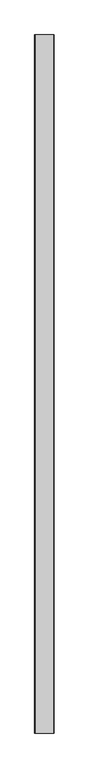
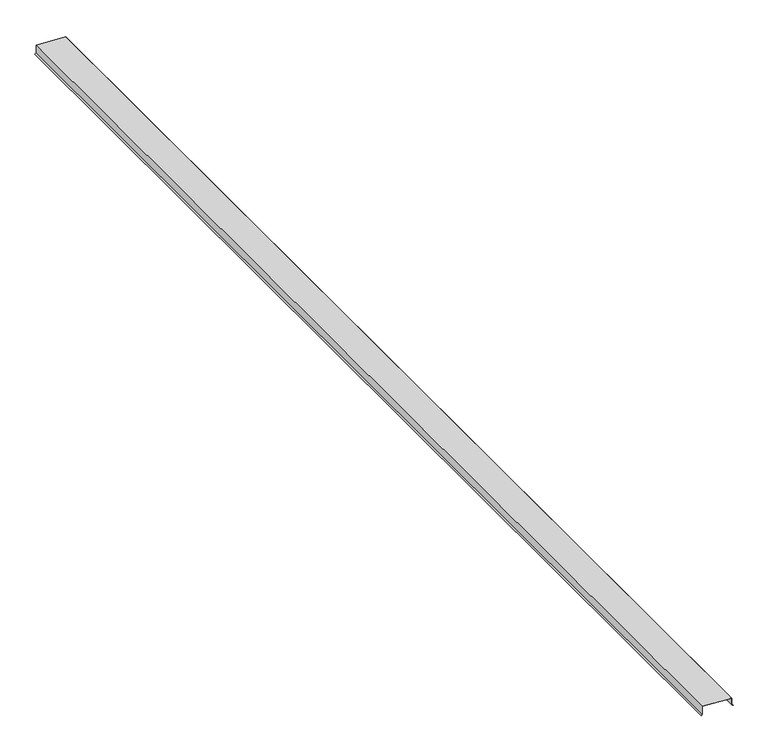
"""IFC4 building model written with IfcOpenShell, lengths in millimetres: proxy geometry, Generic Models 7:Generic Models 1:5:Generic Models 1:5 : Generic Models 7:Generic Models 1:337419:21 : Generic Models 7:Generic Models 1:5:Generic Models 1:5 : Generic Models 7:Generic Models 1:337419:311462."""

from ifc_helpers import new_model, si_unit, frame, origin, place, context, project, spatial, polyline, outline, extrude, source, transform, mapped, element, save


def generic_models_7c79f103(model_context):
    return source(origin(), model_context, "Body", "SweptSolid", [
        extrude(outline(polyline([(6099.8348677, 560254.5367238), (6087.1348677, 560241.8367238), (6086.0123357, 560242.9592559), (6099.1773037, 560256.1242238), (6187.7275706, 560256.1242238), (6171.0881006, 560573.6242239), (6099.1773037, 560573.6242239), (6086.0123357, 560586.7891918), (6087.1348677, 560587.9117239), (6099.8348677, 560575.2117239), (6172.5945819, 560575.2117239), (6189.4004465, 560254.5367238), (6099.8348677, 560254.5367238)])), frame((0.0, -578916.8945489, 0.0), z_axis=(0.0, 1.0, 0.0), x_axis=(0.0, 0.0, 1.0)), (0.0, 0.0, 1.0), 12447.9281647),
    ])


if __name__ == "__main__":
    model = new_model("IFC4")
    model_context = context("Model", 3, world=origin())
    ifc_project = project(units=[si_unit("LENGTHUNIT", "METRE", prefix="MILLI")], contexts=[model_context])
    site = spatial("IfcSite", under=ifc_project)
    building = spatial("IfcBuilding", under=site)
    placement = place(None, origin())
    generic_models_shape = generic_models_7c79f103(model_context)
    element("IfcBuildingElementProxy", 1, Name="Generic Models 7:Generic Models 1:5:Generic Models 1:5 : Generic Models 7:Generic Models 1:337419:21 : Generic Models 7:Generic Models 1:5:Generic Models 1:5 : Generic Models 7:Generic Models 1:337419:311462", ObjectType="Generic Models 7:Generic Models 1:5:Generic Models 1:5 : Generic Models 7:Generic Models 1:337419:21 : Generic Models 7:Generic Models 1:5:Generic Models 1:5 : Generic Models 7:Generic Models 1:337419:311462", at=placement, inside=building, context=model_context, shape_type="MappedRepresentation", body=[
        mapped(generic_models_shape, transform((0.0, 0.0, 0.0), x_axis=(1.0, 0.0, 0.0), y_axis=(0.0, 1.0, 0.0), z_axis=(0.0, 0.0, 1.0))),
    ])
    save(model, "model.ifc")

# Revit data of these elements
# Type "Generic Models 7:Generic Models 1:5:Generic Models 1:5 : Generic Models 7:Generic Models 1:337419:21 : Generic Models 7:Generic Models 1:5:Generic Models 1:5 : Generic Models 7:Generic Models 1:337419:311462"
#   NameOverride = "Generic Models 7:Generic Models 1:5:Generic Models 1:5 : Generic Models 7:Generic Models 1:337419:311462"
#   ObjectTypeOverride = "Generic Models 1:5 : Generic Models 7:Generic Models 1:337419"
#   Reference = "Generic Models 1"
#   Tag = "311462"
# Element 1 (IfcBuildingElementProxy, "Generic Models 7:Generic Models 1:5:Generic Models 1:5 : Generic Models 7:Generic Models 1:337419:21 : Generic Models 7:Generic Models 1:5:Generic Models 1:5 : Generic Models 7:Generic Models 1:337419:311462")
#   Materials on its faces: "SLOPED SHEET METAL COPING - (COLOR TO MATCH RESIN PANEL)"
# Materials
#   "SLOPED SHEET METAL COPING - (COLOR TO MATCH RESIN PANEL)": class "Generic", colour RGB 240 240 240, transparency 0, Keynote = "M07711300.01", Cost = 0
